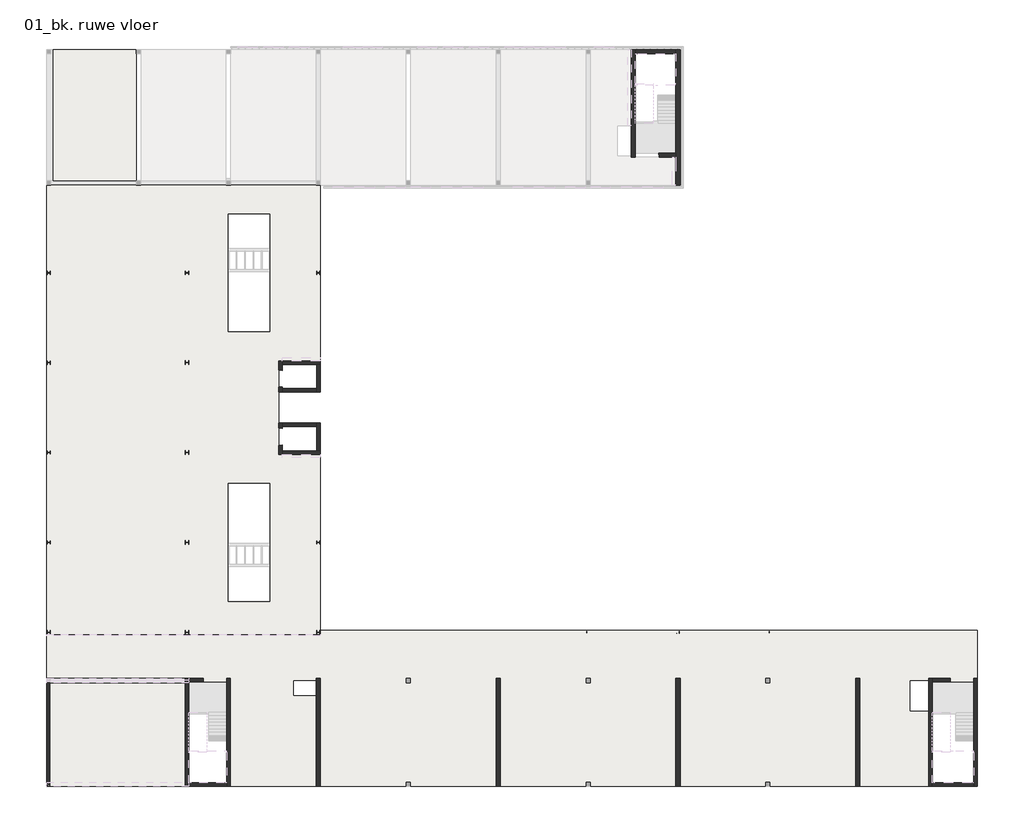
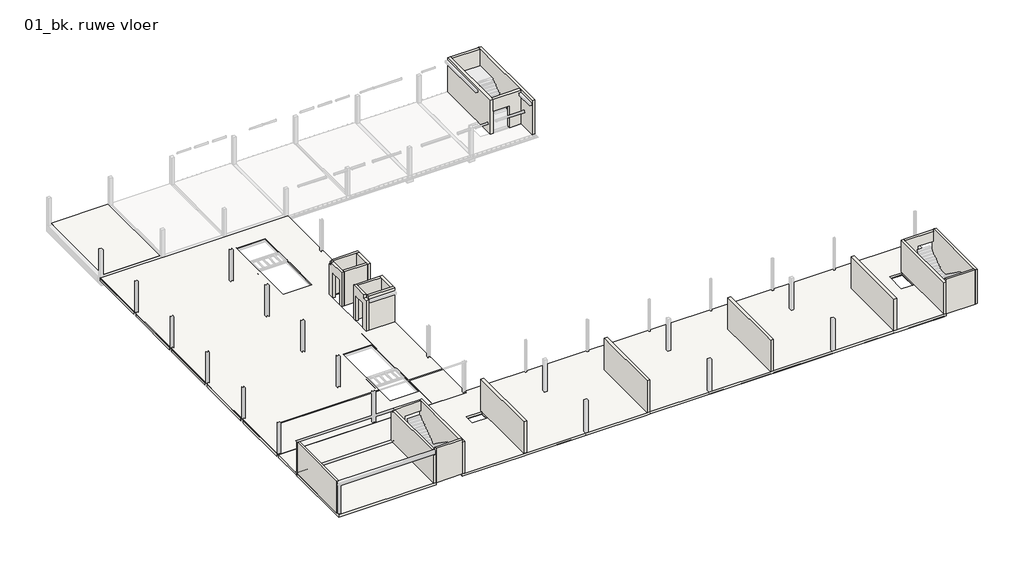
# One storey, part 1 of 4: 25 walls, 20 slabs.
"""IFC4 building model written with IfcOpenShell, lengths in millimetres."""

from ifc_helpers import new_model, si_unit, frame, origin, place, context, project, spatial, polyline, outline, extrude, faceted_brep, element, save

model = new_model("IFC4")

# Units and contexts
model_context = context("Model", 3, world=origin())
ifc_project = project(units=[si_unit("LENGTHUNIT", "METRE", prefix="MILLI")], contexts=[model_context])

# Site, building, storey
site = spatial("IfcSite", under=ifc_project)
building = spatial("IfcBuilding", under=site)
storey = spatial("IfcBuildingStorey", under=building, Name="01_bk. ruwe vloer", Elevation=3730.0)

# Slabs
placement = place(None, origin())
element("IfcSlab", 1, ObjectType="NLRS_23_FL_breedplaat 260_gen_rsf", at=placement, inside=storey, context=model_context, shape_type="Brep", body=[
    faceted_brep([(70375.0, -150.0, 3470.0), (70125.0, -150.0, 3470.0), (65200.0, -150.0, 3470.0), (64800.0, -150.0, 3470.0), (52200.0, -150.0, 3470.0), (51800.0, -150.0, 3470.0), (39200.0, -150.0, 3470.0), (38800.0, -150.0, 3470.0), (26200.0, -150.0, 3470.0), (25800.0, -150.0, 3470.0), (19625.0, -150.0, 3470.0), (19375.0, -150.0, 3470.0), (19375.0, 7400.0, 3470.0), (16625.0, 7400.0, 3470.0), (16625.0, 7493.0, 3470.0), (16625.0, 7507.0, 3470.0), (6350.0, 7507.0, 3470.0), (6350.0, 10845.0, 3470.0), (26125.0, 10845.0, 3470.0), (26125.0, 11125.0, 3470.0), (73650.0, 11125.0, 3470.0), (73650.0, 7400.0, 3470.0), (73400.0, 7400.0, 3470.0), (70375.0, 7400.0, 3470.0), (19600.0, 7622.0, 3470.0), (19600.0, -140.0, 3470.0), (25825.0, -140.0, 3470.0), (25825.0, 125.0, 3470.0), (26175.0, 125.0, 3470.0), (26175.0, -140.0, 3470.0), (32375.0, -140.0, 3470.0), (32375.0, 7625.0, 3470.0), (32625.0, 7625.0, 3470.0), (32625.0, -140.0, 3470.0), (38825.0, -140.0, 3470.0), (38825.0, 125.0, 3470.0), (39175.0, 125.0, 3470.0), (39175.0, -140.0, 3470.0), (45375.0, -140.0, 3470.0), (45375.0, 7625.0, 3470.0), (45625.0, 7625.0, 3470.0), (45625.0, -140.0, 3470.0), (51825.0, -140.0, 3470.0), (51825.0, 125.0, 3470.0), (52175.0, 125.0, 3470.0), (52175.0, -140.0, 3470.0), (58375.0, -140.0, 3470.0), (58375.0, 7625.0, 3470.0), (58625.0, 7625.0, 3470.0), (58625.0, -140.0, 3470.0), (64825.0, -140.0, 3470.0), (64825.0, 125.0, 3470.0), (65175.0, 125.0, 3470.0), (65175.0, -140.0, 3470.0), (70150.0, -140.0, 3470.0), (70150.0, 7625.0, 3470.0), (73640.0, 7625.0, 3470.0), (73640.0, 11115.0, 3470.0), (26135.0, 11115.0, 3470.0), (26135.0, 10750.0, 3470.0), (6360.0, 10750.0, 3470.0), (6360.0, 7622.0, 3470.0), (51825.0, 7625.0, 3470.0), (52175.0, 7625.0, 3470.0), (52175.0, 7375.0, 3470.0), (51825.0, 7375.0, 3470.0), (64825.0, 7625.0, 3470.0), (65175.0, 7625.0, 3470.0), (65175.0, 7375.0, 3470.0), (64825.0, 7375.0, 3470.0), (38825.0, 7625.0, 3470.0), (39175.0, 7625.0, 3470.0), (39175.0, 7375.0, 3470.0), (38825.0, 7375.0, 3470.0), (25850.0, 7375.0, 3470.0), (25850.0, 7500.0, 3470.0), (25825.0, 7500.0, 3470.0), (25825.0, 7625.0, 3470.0), (26175.0, 7625.0, 3470.0), (26175.0, 7375.0, 3470.0), (19375.0, -150.0, 3730.0), (19625.0, -150.0, 3730.0), (25850.0, -150.0, 3730.0), (26150.0, -150.0, 3730.0), (32350.0, -150.0, 3730.0), (32650.0, -150.0, 3730.0), (38850.0, -150.0, 3730.0), (39150.0, -150.0, 3730.0), (45350.0, -150.0, 3730.0), (45650.0, -150.0, 3730.0), (51850.0, -150.0, 3730.0), (52150.0, -150.0, 3730.0), (58350.0, -150.0, 3730.0), (58650.0, -150.0, 3730.0), (64850.0, -150.0, 3730.0), (65150.0, -150.0, 3730.0), (70125.0, -150.0, 3730.0), (70375.0, -150.0, 3730.0), (70375.0, 7400.0, 3730.0), (71700.0, 7400.0, 3730.0), (73650.0, 7400.0, 3730.0), (73650.0, 11125.0, 3730.0), (26125.0, 11125.0, 3730.0), (26125.0, 10845.0, 3730.0), (6350.0, 10845.0, 3730.0), (6350.0, 7507.0, 3730.0), (16625.0, 7507.0, 3730.0), (16625.0, 7493.0, 3730.0), (16625.0, 7400.0, 3730.0), (19375.0, 7400.0, 3730.0), (19375.0, 100.0, 3730.0), (24227.5, 6452.0, 3730.0), (24227.5, 7500.0, 3730.0), (25850.0, 7500.0, 3730.0), (25850.0, 6452.0, 3730.0), (68805.0, 5320.0, 3730.0), (68805.0, 7500.0, 3730.0), (70125.0, 7500.0, 3730.0), (70125.0, 5320.0, 3730.0), (6350.0, 10845.0, 3680.0), (26125.0, 10845.0, 3680.0), (19600.0, -140.0, 3530.0), (19600.0, 7622.0, 3530.0), (6360.0, 7622.0, 3530.0), (6360.0, 10750.0, 3530.0), (26135.0, 10750.0, 3530.0), (26135.0, 11115.0, 3530.0), (73640.0, 11115.0, 3530.0), (73640.0, 7625.0, 3530.0), (70150.0, 7625.0, 3530.0), (70150.0, -140.0, 3530.0), (65175.0, -140.0, 3530.0), (65175.0, 125.0, 3530.0), (64825.0, 125.0, 3530.0), (64825.0, -140.0, 3530.0), (58625.0, -140.0, 3530.0), (58625.0, 7625.0, 3530.0), (58375.0, 7625.0, 3530.0), (58375.0, -140.0, 3530.0), (52175.0, -140.0, 3530.0), (52175.0, 125.0, 3530.0), (51825.0, 125.0, 3530.0), (51825.0, -140.0, 3530.0), (45625.0, -140.0, 3530.0), (45625.0, 7625.0, 3530.0), (45375.0, 7625.0, 3530.0), (45375.0, -140.0, 3530.0), (39175.0, -140.0, 3530.0), (39175.0, 125.0, 3530.0), (38825.0, 125.0, 3530.0), (38825.0, -140.0, 3530.0), (32625.0, -140.0, 3530.0), (32625.0, 7625.0, 3530.0), (32375.0, 7625.0, 3530.0), (32375.0, -140.0, 3530.0), (26175.0, -140.0, 3530.0), (26175.0, 125.0, 3530.0), (25825.0, 125.0, 3530.0), (25825.0, -140.0, 3530.0), (26175.0, 7625.0, 3530.0), (25825.0, 7625.0, 3530.0), (25825.0, 7500.0, 3530.0), (24227.5, 7500.0, 3530.0), (24227.5, 6452.0, 3530.0), (25850.0, 6452.0, 3530.0), (25850.0, 7375.0, 3530.0), (26175.0, 7375.0, 3530.0), (52175.0, 7625.0, 3530.0), (51825.0, 7625.0, 3530.0), (51825.0, 7375.0, 3530.0), (52175.0, 7375.0, 3530.0), (65175.0, 7625.0, 3530.0), (64825.0, 7625.0, 3530.0), (64825.0, 7375.0, 3530.0), (65175.0, 7375.0, 3530.0), (39175.0, 7625.0, 3530.0), (38825.0, 7625.0, 3530.0), (38825.0, 7375.0, 3530.0), (39175.0, 7375.0, 3530.0), (68805.0, 7500.0, 3530.0), (68805.0, 5320.0, 3530.0), (70125.0, 5320.0, 3530.0), (70125.0, 7500.0, 3530.0)], [[[0, 1, 2, 3, 4, 5, 6, 7, 8, 9, 10, 11, 12, 13, 14, 15, 16, 17, 18, 19, 20, 21, 22, 23], [24, 25, 26, 27, 28, 29, 30, 31, 32, 33, 34, 35, 36, 37, 38, 39, 40, 41, 42, 43, 44, 45, 46, 47, 48, 49, 50, 51, 52, 53, 54, 55, 56, 57, 58, 59, 60, 61]], [[62, 63, 64, 65]], [[66, 67, 68, 69]], [[70, 71, 72, 73]], [[74, 75, 76, 77, 78, 79]], [[80, 81, 82, 83, 84, 85, 86, 87, 88, 89, 90, 91, 92, 93, 94, 95, 96, 97, 98, 99, 100, 101, 102, 103, 104, 105, 106, 107, 108, 109, 110], [111, 112, 113, 114], [115, 116, 117, 118]], [[11, 10, 9, 8, 7, 6, 5, 4, 3, 2, 1, 0, 97, 96, 95, 94, 93, 92, 91, 90, 89, 88, 87, 86, 85, 84, 83, 82, 81, 80]], [[12, 11, 80, 110, 109]], [[13, 12, 109, 108]], [[13, 108, 107, 106, 15, 14]], [[17, 16, 105, 104, 119]], [[18, 17, 119, 104, 103, 120]], [[19, 18, 120, 103, 102]], [[20, 19, 102, 101]], [[21, 20, 101, 100]], [[23, 22, 21, 100, 99, 98]], [[0, 23, 98, 97]], [[16, 15, 106, 105]], [[121, 122, 123, 124, 125, 126, 127, 128, 129, 130, 131, 132, 133, 134, 135, 136, 137, 138, 139, 140, 141, 142, 143, 144, 145, 146, 147, 148, 149, 150, 151, 152, 153, 154, 155, 156, 157, 158], [159, 160, 161, 162, 163, 164, 165, 166], [167, 168, 169, 170], [171, 172, 173, 174], [175, 176, 177, 178], [179, 180, 181, 182]], [[122, 121, 25, 24]], [[123, 122, 24, 61]], [[124, 123, 61, 60]], [[125, 124, 60, 59]], [[126, 125, 59, 58]], [[127, 126, 58, 57]], [[128, 127, 57, 56]], [[129, 128, 56, 55]], [[130, 129, 55, 54]], [[131, 130, 54, 53]], [[132, 131, 53, 52]], [[133, 132, 52, 51]], [[134, 133, 51, 50]], [[135, 134, 50, 49]], [[136, 135, 49, 48]], [[137, 136, 48, 47]], [[138, 137, 47, 46]], [[139, 138, 46, 45]], [[140, 139, 45, 44]], [[141, 140, 44, 43]], [[142, 141, 43, 42]], [[143, 142, 42, 41]], [[144, 143, 41, 40]], [[145, 144, 40, 39]], [[146, 145, 39, 38]], [[147, 146, 38, 37]], [[148, 147, 37, 36]], [[149, 148, 36, 35]], [[150, 149, 35, 34]], [[151, 150, 34, 33]], [[152, 151, 33, 32]], [[153, 152, 32, 31]], [[154, 153, 31, 30]], [[155, 154, 30, 29]], [[156, 155, 29, 28]], [[157, 156, 28, 27]], [[158, 157, 27, 26]], [[121, 158, 26, 25]], [[160, 159, 78, 77]], [[161, 160, 77, 76]], [[166, 165, 74, 79]], [[159, 166, 79, 78]], [[168, 167, 63, 62]], [[169, 168, 62, 65]], [[170, 169, 65, 64]], [[167, 170, 64, 63]], [[172, 171, 67, 66]], [[173, 172, 66, 69]], [[174, 173, 69, 68]], [[171, 174, 68, 67]], [[176, 175, 71, 70]], [[177, 176, 70, 73]], [[178, 177, 73, 72]], [[175, 178, 72, 71]], [[112, 111, 163, 162]], [[111, 114, 164, 163]], [[113, 75, 74, 165, 164, 114]], [[75, 113, 112, 162, 161, 76]], [[116, 115, 180, 179]], [[115, 118, 181, 180]], [[118, 117, 182, 181]], [[117, 116, 179, 182]]]),
])
element("IfcSlab", 2, ObjectType="NLRS_23_FL_breedplaat 260_gen_rsf", at=placement, inside=storey, context=model_context, shape_type="Brep", body=[
    faceted_brep([(6830.0, 43680.0, 3470.0), (6830.0, 43800.0, 3470.0), (6830.0, 53150.0, 3470.0), (6950.0, 53150.0, 3470.0), (12700.0, 53150.0, 3470.0), (12820.0, 53150.0, 3470.0), (12820.0, 43680.0, 3470.0), (12700.0, 43680.0, 3470.0), (12725.0, 43775.0, 3470.0), (12725.0, 53140.0, 3470.0), (6925.0, 53140.0, 3470.0), (6925.0, 43775.0, 3470.0), (6830.0, 53150.0, 3730.0), (6830.0, 43680.0, 3730.0), (12820.0, 43680.0, 3730.0), (12820.0, 53150.0, 3730.0), (6925.0, 53140.0, 3530.0), (12725.0, 53140.0, 3530.0), (12725.0, 43775.0, 3530.0), (6925.0, 43775.0, 3530.0)], [[[0, 1, 2, 3, 4, 5, 6, 7], [8, 9, 10, 11]], [[12, 13, 14, 15]], [[2, 1, 0, 13, 12]], [[5, 4, 3, 2, 12, 15]], [[6, 5, 15, 14]], [[0, 7, 6, 14, 13]], [[16, 17, 18, 19]], [[18, 17, 9, 8]], [[19, 18, 8, 11]], [[16, 19, 11, 10]], [[17, 16, 10, 9]]]),
])
element("IfcSlab", 3, ObjectType="NLRS_23_FL_druklaag 70_gen_rsf", at=placement, inside=storey, context=model_context, shape_type="Brep", body=[
    faceted_brep([(26125.0, 23875.0, 3660.0), (26125.0, 23795.0, 3660.0), (26125.0, 17675.0, 3660.0), (26125.0, 17655.0, 3660.0), (26125.0, 17345.0, 3660.0), (26125.0, 17325.0, 3660.0), (26125.0, 11175.0, 3660.0), (26125.0, 11155.0, 3660.0), (6350.0, 11155.0, 3660.0), (6350.0, 11175.0, 3660.0), (6350.0, 17325.0, 3660.0), (6350.0, 17345.0, 3660.0), (19240.0, 17345.0, 3660.0), (19240.0, 17655.0, 3660.0), (6350.0, 17655.0, 3660.0), (6350.0, 17675.0, 3660.0), (6350.0, 23825.0, 3660.0), (6350.0, 23845.0, 3660.0), (19240.0, 23845.0, 3660.0), (19500.0, 23845.0, 3660.0), (22500.0, 23845.0, 3660.0), (22760.0, 23845.0, 3660.0), (23362.3, 23845.0, 3660.0), (23362.3, 23875.0, 3660.0), (22500.0, 21750.0, 3660.0), (19500.0, 21750.0, 3660.0), (19500.0, 13250.0, 3660.0), (22500.0, 13250.0, 3660.0), (19500.0000006, 22062.0, 3660.0), (19500.0000006, 21760.0, 3660.0), (22499.9999994, 21760.0, 3660.0), (22499.9999994, 22062.0, 3660.0), (19500.0000006, 13240.0, 3660.0), (19500.0000006, 12938.0, 3660.0), (22499.9999994, 12938.0, 3660.0), (22499.9999994, 13240.0, 3660.0), (23125.0, 24155.0, 3660.0), (6350.0, 24155.0, 3660.0), (6350.0, 24175.0, 3660.0), (6350.0, 30302.0, 3660.0), (6350.0, 30322.0, 3660.0), (23125.0, 30322.0, 3660.0), (23125.0, 30302.0, 3660.0), (23125.0, 24175.0, 3660.0), (6350.0, 43350.0, 3660.0), (26125.0, 43350.0, 3660.0), (26125.0, 43330.0, 3660.0), (26125.0, 37175.0, 3660.0), (26125.0, 37155.0, 3660.0), (22760.0, 37155.0, 3660.0), (22760.0, 36845.0, 3660.0), (26125.0, 36845.0, 3660.0), (26125.0, 36825.0, 3660.0), (26125.0, 30705.0, 3660.0), (26125.0, 30625.0, 3660.0), (23362.3, 30625.0, 3660.0), (23362.3, 30632.0, 3660.0), (6350.0, 30632.0, 3660.0), (6350.0, 30652.0, 3660.0), (6350.0, 36825.0, 3660.0), (6350.0, 36845.0, 3660.0), (19240.0, 36845.0, 3660.0), (19240.0, 37155.0, 3660.0), (6350.0, 37155.0, 3660.0), (6350.0, 37175.0, 3660.0), (6350.0, 43330.0, 3660.0), (22500.0, 32750.0, 3660.0), (22500.0, 41250.0, 3660.0), (19500.0, 41250.0, 3660.0), (19500.0, 32750.0, 3660.0), (19500.0000006, 41562.0, 3660.0), (19500.0000006, 41260.0, 3660.0), (22499.9999994, 41260.0, 3660.0), (22499.9999994, 41562.0, 3660.0), (19500.0000006, 32740.0, 3660.0), (19500.0000006, 32438.0, 3660.0), (22499.9999994, 32438.0, 3660.0), (22499.9999994, 32740.0, 3660.0), (26125.0, 30625.0, 3730.0), (26125.0, 43350.0, 3730.0), (13180.0, 43350.0, 3730.0), (12820.0, 43350.0, 3730.0), (6350.0, 43350.0, 3730.0), (6350.0, 10845.0, 3730.0), (26125.0, 10845.0, 3730.0), (26125.0, 11125.0, 3730.0), (26125.0, 23875.0, 3730.0), (23125.0, 23875.0, 3730.0), (23125.0, 30625.0, 3730.0), (22500.0, 41250.0, 3730.0), (22500.0, 32750.0, 3730.0), (19500.0, 32750.0, 3730.0), (19500.0, 41250.0, 3730.0), (19500.0, 21750.0, 3730.0), (22500.0, 21750.0, 3730.0), (22500.0, 13250.0, 3730.0), (19500.0, 13250.0, 3730.0), (26125.0, 36845.0, 3680.0), (26125.0, 37155.0, 3680.0), (6350.0, 10845.0, 3680.0), (26125.0, 10845.0, 3680.0), (6350.0, 37155.0, 3680.0), (6350.0, 36845.0, 3680.0), (6350.0, 30632.0, 3680.0), (6350.0, 30322.0, 3680.0), (6350.0, 24155.0, 3680.0), (6350.0, 23845.0, 3680.0), (6350.0, 17655.0, 3680.0), (6350.0, 17345.0, 3680.0), (6350.0, 11155.0, 3680.0), (23125.0, 30625.0, 3680.0), (23362.3, 30625.0, 3680.0), (23125.0, 23875.0, 3680.0), (23125.0, 24155.0, 3680.0), (23125.0, 30322.0, 3680.0), (23362.3, 23875.0, 3680.0), (26125.0, 11125.0, 3680.0), (26125.0, 11155.0, 3680.0), (19240.0, 17345.0, 3680.0), (19240.0, 17655.0, 3680.0), (23362.3, 23845.0, 3680.0), (23362.3, 30632.0, 3680.0), (19240.0, 36845.0, 3680.0), (19240.0, 37155.0, 3680.0), (22760.0, 37155.0, 3680.0), (22760.0, 36845.0, 3680.0), (19500.0000006, 41562.0, 3680.0), (19500.0000006, 41260.0, 3680.0), (22499.9999994, 41260.0, 3680.0), (22499.9999994, 41562.0, 3680.0), (19500.0000006, 32740.0, 3680.0), (19500.0000006, 32438.0, 3680.0), (22499.9999994, 32438.0, 3680.0), (22499.9999994, 32740.0, 3680.0), (19500.0000006, 22062.0, 3680.0), (19500.0000006, 21760.0, 3680.0), (22499.9999994, 21760.0, 3680.0), (22499.9999994, 22062.0, 3680.0), (19500.0000006, 13240.0, 3680.0), (19500.0000006, 12938.0, 3680.0), (22499.9999994, 12938.0, 3680.0), (22499.9999994, 13240.0, 3680.0)], [[[0, 1, 2, 3, 4, 5, 6, 7, 8, 9, 10, 11, 12, 13, 14, 15, 16, 17, 18, 19, 20, 21, 22, 23], [24, 25, 26, 27], [28, 29, 30, 31], [32, 33, 34, 35]], [[36, 37, 38, 39, 40, 41, 42, 43]], [[44, 45, 46, 47, 48, 49, 50, 51, 52, 53, 54, 55, 56, 57, 58, 59, 60, 61, 62, 63, 64, 65], [66, 67, 68, 69], [70, 71, 72, 73], [74, 75, 76, 77]], [[78, 79, 80, 81, 82, 83, 84, 85, 86, 87, 88], [89, 90, 91, 92], [93, 94, 95, 96]], [[79, 78, 54, 53, 52, 51, 97, 98, 48, 47, 46, 45]], [[84, 83, 99, 100]], [[83, 82, 44, 65, 64, 63, 101, 102, 60, 59, 58, 57, 103, 104, 40, 39, 38, 37, 105, 106, 17, 16, 15, 14, 107, 108, 11, 10, 9, 8, 109, 99]], [[45, 44, 82, 81, 80, 79]], [[78, 88, 110, 111, 55, 54]], [[88, 87, 112, 113, 36, 43, 42, 41, 114, 110]], [[87, 86, 0, 23, 115, 112]], [[0, 86, 85, 84, 100, 116, 117, 7, 6, 5, 4, 3, 2, 1]], [[67, 66, 90, 89]], [[68, 67, 89, 92]], [[69, 68, 92, 91]], [[66, 69, 91, 90]], [[25, 24, 94, 93]], [[26, 25, 93, 96]], [[27, 26, 96, 95]], [[24, 27, 95, 94]], [[109, 117, 116, 100, 99]], [[117, 109, 8, 7]], [[118, 119, 13, 12]], [[119, 118, 108, 107]], [[119, 107, 14, 13]], [[108, 118, 12, 11]], [[120, 115, 23, 22]], [[120, 106, 105, 113, 112, 115]], [[113, 105, 37, 36]], [[106, 120, 22, 21, 20, 19, 18, 17]], [[111, 121, 56, 55]], [[103, 121, 111, 110, 114, 104]], [[121, 103, 57, 56]], [[104, 114, 41, 40]], [[122, 123, 62, 61]], [[123, 122, 102, 101]], [[123, 101, 63, 62]], [[102, 122, 61, 60]], [[124, 125, 50, 49]], [[125, 124, 98, 97]], [[98, 124, 49, 48]], [[125, 97, 51, 50]], [[126, 127, 71, 70]], [[128, 129, 73, 72]], [[127, 126, 129, 128]], [[127, 128, 72, 71]], [[129, 126, 70, 73]], [[130, 131, 75, 74]], [[132, 133, 77, 76]], [[131, 130, 133, 132]], [[133, 130, 74, 77]], [[131, 132, 76, 75]], [[134, 135, 29, 28]], [[136, 137, 31, 30]], [[135, 134, 137, 136]], [[135, 136, 30, 29]], [[137, 134, 28, 31]], [[138, 139, 33, 32]], [[140, 141, 35, 34]], [[139, 138, 141, 140]], [[141, 138, 32, 35]], [[139, 140, 34, 33]]]),
])
element("IfcSlab", 4, ObjectType="NLRS_23_FL_kanaalplaat 260_gen_rsf", at=placement, inside=storey, context=model_context, shape_type="SweptSolid", body=[
    extrude(outline(polyline([(19240.0, 11175.0), (6350.0, 11175.0), (6350.0, 17325.0), (19240.0, 17325.0), (19240.0, 11175.0)])), frame((0.0, 0.0, 3400.0), z_axis=(0.0, 0.0, 1.0), x_axis=(1.0, 0.0, 0.0)), (0.0, 0.0, 1.0), 260.0),
])
element("IfcSlab", 5, ObjectType="NLRS_23_FL_kanaalplaat 260_gen_rsf", at=placement, inside=storey, context=model_context, shape_type="SweptSolid", body=[
    extrude(outline(polyline([(6350.0, 17675.0), (6350.0, 23825.0), (19240.0, 23825.0), (19240.0, 17675.0), (6350.0, 17675.0)])), frame((0.0, 0.0, 3400.0), z_axis=(0.0, 0.0, 1.0), x_axis=(1.0, 0.0, 0.0)), (0.0, 0.0, 1.0), 260.0),
])
element("IfcSlab", 6, ObjectType="NLRS_23_FL_kanaalplaat 260_gen_rsf", at=placement, inside=storey, context=model_context, shape_type="SweptSolid", body=[
    extrude(outline(polyline([(23125.0, 30302.0), (23125.0, 24175.0), (6350.0, 24175.0), (6350.0, 30302.0), (23125.0, 30302.0)])), frame((0.0, 0.0, 3400.0), z_axis=(0.0, 0.0, 1.0), x_axis=(1.0, 0.0, 0.0)), (0.0, 0.0, 1.0), 260.0),
])
element("IfcSlab", 7, ObjectType="NLRS_23_FL_kanaalplaat 260_gen_rsf", at=placement, inside=storey, context=model_context, shape_type="SweptSolid", body=[
    extrude(outline(polyline([(22500.0, 23825.0), (22500.0, 22082.0), (19500.0, 22082.0), (19500.0, 23825.0), (22500.0, 23825.0)])), frame((0.0, 0.0, 3400.0), z_axis=(0.0, 0.0, 1.0), x_axis=(1.0, 0.0, 0.0)), (0.0, 0.0, 1.0), 260.0),
])
element("IfcSlab", 8, ObjectType="NLRS_23_FL_kanaalplaat 260_gen_rsf", at=placement, inside=storey, context=model_context, shape_type="SweptSolid", body=[
    extrude(outline(polyline([(22500.0, 11182.5), (19500.0, 11182.5), (19500.0, 12918.0), (22500.0, 12918.0), (22500.0, 11182.5)])), frame((0.0, 0.0, 3400.0), z_axis=(0.0, 0.0, 1.0), x_axis=(1.0, 0.0, 0.0)), (0.0, 0.0, 1.0), 260.0),
])
element("IfcSlab", 9, ObjectType="NLRS_23_FL_kanaalplaat 260_gen_rsf", at=placement, inside=storey, context=model_context, shape_type="Brep", body=[
    faceted_brep([(26125.0, 23795.0, 3400.0), (26125.0, 23625.0, 3400.0), (26125.0, 17675.0, 3400.0), (22760.0, 17675.0, 3400.0), (22760.0, 23825.0, 3400.0), (23395.0, 23825.0, 3400.0), (23395.0, 23795.0, 3400.0), (26125.0, 23795.0, 3660.0), (23395.0, 23795.0, 3660.0), (23395.0, 23825.0, 3660.0), (22760.0, 23825.0, 3660.0), (22760.0, 17675.0, 3660.0), (26125.0, 17675.0, 3660.0)], [[[0, 1, 2, 3, 4, 5, 6]], [[7, 8, 9, 10, 11, 12]], [[2, 1, 0, 7, 12]], [[3, 2, 12, 11]], [[4, 3, 11, 10]], [[5, 4, 10, 9]], [[6, 5, 9, 8]], [[0, 6, 8, 7]]]),
])
element("IfcSlab", 10, ObjectType="NLRS_23_FL_kanaalplaat 260_gen_rsf", at=placement, inside=storey, context=model_context, shape_type="SweptSolid", body=[
    extrude(outline(polyline([(22760.0, 11175.0), (22760.0, 17325.0), (26125.0, 17325.0), (26125.0, 11175.0), (22760.0, 11175.0)])), frame((0.0, 0.0, 3400.0), z_axis=(0.0, 0.0, 1.0), x_axis=(1.0, 0.0, 0.0)), (0.0, 0.0, 1.0), 260.0),
])
element("IfcSlab", 11, ObjectType="NLRS_23_FL_kanaalplaat 260_gen_rsf", at=placement, inside=storey, context=model_context, shape_type="Brep", body=[
    faceted_brep([(19240.0, 43330.0, 3400.0), (19240.0, 37175.0, 3400.0), (6350.0, 37175.0, 3400.0), (6350.0, 43200.0, 3400.0), (6350.0, 43330.0, 3400.0), (19240.0, 43330.0, 3660.0), (6350.0, 43330.0, 3660.0), (6350.0, 37175.0, 3660.0), (19240.0, 37175.0, 3660.0)], [[[0, 1, 2, 3, 4]], [[5, 6, 7, 8]], [[0, 4, 6, 5]], [[4, 3, 2, 7, 6]], [[2, 1, 8, 7]], [[1, 0, 5, 8]]]),
])
element("IfcSlab", 12, ObjectType="NLRS_23_FL_kanaalplaat 260_gen_rsf", at=placement, inside=storey, context=model_context, shape_type="SweptSolid", body=[
    extrude(outline(polyline([(6350.0, 36825.0), (19240.0, 36825.0), (19240.0, 30652.0), (6350.0, 30652.0), (6350.0, 36825.0)])), frame((0.0, 0.0, 3400.0), z_axis=(0.0, 0.0, 1.0), x_axis=(1.0, 0.0, 0.0)), (0.0, 0.0, 1.0), 260.0),
])
element("IfcSlab", 13, ObjectType="NLRS_23_FL_kanaalplaat 260_gen_rsf", at=placement, inside=storey, context=model_context, shape_type="SweptSolid", body=[
    extrude(outline(polyline([(22500.0, 30652.0), (19500.0, 30652.0), (19500.0, 32418.0), (22500.0, 32418.0), (22500.0, 30652.0)])), frame((0.0, 0.0, 3400.0), z_axis=(0.0, 0.0, 1.0), x_axis=(1.0, 0.0, 0.0)), (0.0, 0.0, 1.0), 260.0),
])
element("IfcSlab", 14, ObjectType="NLRS_23_FL_kanaalplaat 260_gen_rsf", at=placement, inside=storey, context=model_context, shape_type="SweptSolid", body=[
    extrude(outline(polyline([(22500.0, 43330.0), (22500.0, 41582.0), (19500.0, 41582.0), (19500.0, 43330.0), (22500.0, 43330.0)])), frame((0.0, 0.0, 3400.0), z_axis=(0.0, 0.0, 1.0), x_axis=(1.0, 0.0, 0.0)), (0.0, 0.0, 1.0), 260.0),
])
element("IfcSlab", 15, ObjectType="NLRS_23_FL_kanaalplaat 260_gen_rsf", at=placement, inside=storey, context=model_context, shape_type="Brep", body=[
    faceted_brep([(26125.0, 30705.0, 3400.0), (23395.0, 30705.0, 3400.0), (23395.0, 30652.0, 3400.0), (22760.0, 30652.0, 3400.0), (22760.0, 36825.0, 3400.0), (26125.0, 36825.0, 3400.0), (26125.0, 30875.0, 3400.0), (26125.0, 30705.0, 3660.0), (26125.0, 36825.0, 3660.0), (22760.0, 36825.0, 3660.0), (22760.0, 30652.0, 3660.0), (23395.0, 30652.0, 3660.0), (23395.0, 30705.0, 3660.0)], [[[0, 1, 2, 3, 4, 5, 6]], [[7, 8, 9, 10, 11, 12]], [[0, 6, 5, 8, 7]], [[5, 4, 9, 8]], [[4, 3, 10, 9]], [[3, 2, 11, 10]], [[2, 1, 12, 11]], [[1, 0, 7, 12]]]),
])
element("IfcSlab", 16, ObjectType="NLRS_23_FL_kanaalplaat 260_gen_rsf", at=placement, inside=storey, context=model_context, shape_type="Brep", body=[
    faceted_brep([(22760.0, 43330.0, 3400.0), (26125.0, 43330.0, 3400.0), (26125.0, 43200.0, 3400.0), (26125.0, 37175.0, 3400.0), (22760.0, 37175.0, 3400.0), (22760.0, 43330.0, 3660.0), (22760.0, 37175.0, 3660.0), (26125.0, 37175.0, 3660.0), (26125.0, 43330.0, 3660.0)], [[[0, 1, 2, 3, 4]], [[5, 6, 7, 8]], [[0, 4, 6, 5]], [[4, 3, 7, 6]], [[3, 2, 1, 8, 7]], [[1, 0, 5, 8]]]),
])
element("IfcSlab", 17, ObjectType="NLRS_23_FL_breedplaat 260_gen_rsf", at=placement, inside=storey, context=model_context, shape_type="Brep", body=[
    faceted_brep([(6350.0, -150.0, 3470.0), (6350.0, 7493.0, 3470.0), (16625.0, 7493.0, 3470.0), (16625.0, -150.0, 3470.0), (6539.0, 125.0, 3470.0), (16400.0, 125.0, 3470.0), (16400.0, 7378.0, 3470.0), (6539.0, 7378.0, 3470.0), (6350.0, 7493.0, 3730.0), (6350.0, -150.0, 3730.0), (16375.0, -150.0, 3730.0), (16625.0, -150.0, 3730.0), (16625.0, 100.0, 3730.0), (16625.0, 7493.0, 3730.0), (16400.0, 7378.0, 3530.0), (16400.0, 125.0, 3530.0), (6539.0, 125.0, 3530.0), (6539.0, 7378.0, 3530.0)], [[[0, 1, 2, 3], [4, 5, 6, 7]], [[8, 9, 10, 11, 12, 13]], [[1, 0, 9, 8]], [[2, 1, 8, 13]], [[3, 2, 13, 12, 11]], [[0, 3, 11, 10, 9]], [[14, 15, 16, 17]], [[16, 15, 5, 4]], [[17, 16, 4, 7]], [[14, 17, 7, 6]], [[15, 14, 6, 5]]]),
])
element("IfcSlab", 18, ObjectType="NLRS_23_FL_breedplaat schil 60_gen_rsf", at=placement, inside=storey, context=model_context, shape_type="SweptSolid", body=[
    extrude(outline(polyline([(16400.0, 125.0), (6539.0, 125.0), (6539.0, 7378.0), (16400.0, 7378.0), (16400.0, 125.0)])), frame((0.0, 0.0, 3470.0), z_axis=(0.0, 0.0, 1.0), x_axis=(1.0, 0.0, 0.0)), (0.0, 0.0, 1.0), 60.0),
])
element("IfcSlab", 19, ObjectType="NLRS_23_FL_breedplaat schil 60_gen_rsf", at=placement, inside=storey, context=model_context, shape_type="SweptSolid", body=[
    extrude(outline(polyline([(19600.0, -140.0), (19600.0, 7622.0), (6360.0, 7622.0), (6360.0, 10750.0), (26135.0, 10750.0), (26135.0, 11115.0), (73640.0, 11115.0), (73640.0, 7625.0), (70150.0, 7625.0), (70150.0, -140.0), (65175.0, -140.0), (65175.0, 125.0), (64825.0, 125.0), (64825.0, -140.0), (58625.0, -140.0), (58625.0, 7625.0), (58375.0, 7625.0), (58375.0, -140.0), (52175.0, -140.0), (52175.0, 125.0), (51825.0, 125.0), (51825.0, -140.0), (45625.0, -140.0), (45625.0, 7625.0), (45375.0, 7625.0), (45375.0, -140.0), (39175.0, -140.0), (39175.0, 125.0), (38825.0, 125.0), (38825.0, -140.0), (32625.0, -140.0), (32625.0, 7625.0), (32375.0, 7625.0), (32375.0, -140.0), (26175.0, -140.0), (26175.0, 125.0), (25825.0, 125.0), (25825.0, -140.0), (19600.0, -140.0)]), holes=[polyline([(26175.0, 7625.0), (25825.0, 7625.0), (25825.0, 7500.0), (24227.5, 7500.0), (24227.5, 6452.0), (25850.0, 6452.0), (25850.0, 7375.0), (26175.0, 7375.0), (26175.0, 7625.0)]), polyline([(52175.0, 7625.0), (51825.0, 7625.0), (51825.0, 7375.0), (52175.0, 7375.0), (52175.0, 7625.0)]), polyline([(65175.0, 7625.0), (64825.0, 7625.0), (64825.0, 7375.0), (65175.0, 7375.0), (65175.0, 7625.0)]), polyline([(39175.0, 7625.0), (38825.0, 7625.0), (38825.0, 7375.0), (39175.0, 7375.0), (39175.0, 7625.0)]), polyline([(68805.0, 7500.0), (68805.0, 5320.0), (70125.0, 5320.0), (70125.0, 7500.0), (68805.0, 7500.0)])]), frame((0.0, 0.0, 3470.0), z_axis=(0.0, 0.0, 1.0), x_axis=(1.0, 0.0, 0.0)), (0.0, 0.0, 1.0), 60.0),
])
element("IfcSlab", 20, ObjectType="NLRS_23_FL_breedplaat schil 60_gen_rsf", at=placement, inside=storey, context=model_context, shape_type="SweptSolid", body=[
    extrude(outline(polyline([(12725.0, 53140.0), (12725.0, 43775.0), (6925.0, 43775.0), (6925.0, 53140.0), (12725.0, 53140.0)])), frame((0.0, 0.0, 3470.0), z_axis=(0.0, 0.0, 1.0), x_axis=(1.0, 0.0, 0.0)), (0.0, 0.0, 1.0), 60.0),
])

# Walls
element("IfcWall", 21, ObjectType="NLRS_22_WA_beton ihw 250_gen_rsf", at=placement, inside=storey, context=model_context, shape_type="Brep", body=[
    faceted_brep([(19625.0, -150.0, 3730.0), (19625.0, 7650.0, 3730.0), (19625.0, 7650.0, 7270.0), (19625.0, -150.0, 7270.0), (19375.0, -150.0, 3730.0), (19375.0, -150.0, 7270.0), (19375.0, 7400.0, 7270.0), (19375.0, 7650.0, 7270.0), (19375.0, 7650.0, 6170.0), (19375.0, 7650.0, 3730.0), (19375.0, 7400.0, 3730.0), (19375.0, 100.0, 3730.0)], [[[0, 1, 2, 3]], [[4, 5, 6, 7, 8, 9, 10, 11]], [[1, 0, 4, 11, 10, 9]], [[2, 1, 9, 8, 7]], [[3, 2, 7, 6, 5]], [[0, 3, 5, 4]]]),
])
element("IfcWall", 22, ObjectType="NLRS_22_WA_beton ihw 250_gen_rsf", at=placement, inside=storey, context=model_context, shape_type="Brep", body=[
    faceted_brep([(16625.0, -150.0, 3730.0), (16625.0, 100.0, 3730.0), (16625.0, 7400.0, 3730.0), (16625.0, 7493.0, 3730.0), (16625.0, 7650.0, 3730.0), (16625.0, 7650.0, 7120.0), (16625.0, 7330.0, 7120.0), (16625.0, 7330.0, 7270.0), (16625.0, 170.0, 7270.0), (16625.0, 170.0, 6880.0), (16625.0, -150.0, 6880.0), (16375.0, -150.0, 3730.0), (16375.0, -150.0, 6880.0), (16375.0, 170.0, 6880.0), (16375.0, 170.0, 7270.0), (16375.0, 7330.0, 7270.0), (16375.0, 7330.0, 7120.0), (16375.0, 7650.0, 7120.0), (16375.0, 7650.0, 3730.0)], [[[0, 1, 2, 3, 4, 5, 6, 7, 8, 9, 10]], [[11, 12, 13, 14, 15, 16, 17, 18]], [[4, 3, 2, 1, 0, 11, 18]], [[5, 4, 18, 17]], [[8, 7, 15, 14]], [[0, 10, 12, 11]], [[6, 5, 17, 16]], [[7, 6, 16, 15]], [[9, 8, 14, 13]], [[10, 9, 13, 12]]]),
])
element("IfcWall", 23, ObjectType="NLRS_22_WA_beton ihw 300_gen_rsf", at=placement, inside=storey, context=model_context, shape_type="Brep", body=[
    faceted_brep([(26150.0, -150.0, 3730.0), (26150.0, 7650.0, 3730.0), (26150.0, 7650.0, 7270.0), (26150.0, -150.0, 7270.0), (25850.0, -150.0, 3730.0), (25850.0, -150.0, 7270.0), (25850.0, 7650.0, 7270.0), (25850.0, 7650.0, 3730.0), (25850.0, 7500.0, 3730.0), (25850.0, 6452.0, 3730.0)], [[[0, 1, 2, 3]], [[4, 5, 6, 7, 8, 9]], [[1, 0, 4, 9, 8, 7]], [[2, 1, 7, 6]], [[3, 2, 6, 5]], [[0, 3, 5, 4]]]),
])
element("IfcWall", 24, ObjectType="NLRS_22_WA_beton ihw 300_gen_rsf", at=placement, inside=storey, context=model_context, shape_type="SweptSolid", body=[
    extrude(outline(polyline([(39150.0, 7650.0), (39150.0, -150.0), (38850.0, -150.0), (38850.0, 7650.0), (39150.0, 7650.0)])), frame((0.0, 0.0, 3730.0), z_axis=(0.0, 0.0, 1.0), x_axis=(1.0, 0.0, 0.0)), (0.0, 0.0, 1.0), 3540.0),
])
element("IfcWall", 25, ObjectType="NLRS_22_WA_beton ihw 300_gen_rsf", at=placement, inside=storey, context=model_context, shape_type="SweptSolid", body=[
    extrude(outline(polyline([(52150.0, 7650.0), (52150.0, -150.0), (51850.0, -150.0), (51850.0, 7650.0), (52150.0, 7650.0)])), frame((0.0, 0.0, 3730.0), z_axis=(0.0, 0.0, 1.0), x_axis=(1.0, 0.0, 0.0)), (0.0, 0.0, 1.0), 3540.0),
])
element("IfcWall", 26, ObjectType="NLRS_22_WA_beton ihw 300_gen_rsf", at=placement, inside=storey, context=model_context, shape_type="SweptSolid", body=[
    extrude(outline(polyline([(65150.0, 7650.0), (65150.0, -150.0), (64850.0, -150.0), (64850.0, 7650.0), (65150.0, 7650.0)])), frame((0.0, 0.0, 3730.0), z_axis=(0.0, 0.0, 1.0), x_axis=(1.0, 0.0, 0.0)), (0.0, 0.0, 1.0), 3540.0),
])
element("IfcWall", 27, ObjectType="NLRS_21_WA_beton ihw 250_gen_rsf", at=placement, inside=storey, context=model_context, shape_type="Brep", body=[
    faceted_brep([(73650.0, -150.0, 3730.0), (73650.0, 7400.0, 3730.0), (73650.0, 7650.0, 3730.0), (73650.0, 7650.0, 7270.0), (73650.0, 7400.0, 7270.0), (73650.0, 7400.0, 7530.0), (73650.0, -150.0, 7530.0), (73400.0, -150.0, 3730.0), (73400.0, -150.0, 7530.0), (73400.0, 100.0, 7530.0), (73400.0, 7400.0, 7530.0), (73400.0, 7400.0, 7270.0), (73400.0, 7650.0, 7270.0), (73400.0, 7650.0, 6170.0), (73400.0, 7650.0, 3730.0), (73400.0, 7400.0, 3730.0), (73400.0, 100.0, 3730.0)], [[[0, 1, 2, 3, 4, 5, 6]], [[7, 8, 9, 10, 11, 12, 13, 14, 15, 16]], [[2, 1, 0, 7, 16, 15, 14]], [[3, 2, 14, 13, 12]], [[6, 5, 10, 9, 8]], [[0, 6, 8, 7]], [[4, 3, 12, 11]], [[5, 4, 11, 10]]]),
])
element("IfcWall", 28, ObjectType="NLRS_21_WA_kalkzandsteen CS12 214_gen_rsf", at=placement, inside=storey, context=model_context, shape_type="SweptSolid", body=[
    extrude(outline(polyline([(6564.0, 7330.0), (6564.0, 170.0), (6350.0, 170.0), (6350.0, 7330.0), (6564.0, 7330.0)])), frame((0.0, 0.0, 3730.0), z_axis=(0.0, 0.0, 1.0), x_axis=(1.0, 0.0, 0.0)), (0.0, 0.0, 1.0), 3540.0),
])
element("IfcWall", 29, ObjectType="NLRS_21_WA_beton ihw 250_gen_rsf", at=placement, inside=storey, context=model_context, shape_type="Brep", body=[
    faceted_brep([(16625.0, -150.0, 3730.0), (19375.0, -150.0, 3730.0), (19375.0, -150.0, 7270.0), (19375.0, -150.0, 7530.0), (16625.0, -150.0, 7530.0), (16625.0, -150.0, 7270.0), (16625.0, -150.0, 6880.0), (19375.0, 100.0, 3730.0), (16625.0, 100.0, 3730.0), (16625.0, 100.0, 7530.0), (19375.0, 100.0, 7530.0), (19375.0, 100.0, 7270.0)], [[[0, 1, 2, 3, 4, 5, 6]], [[7, 8, 9, 10, 11]], [[1, 0, 8, 7]], [[1, 7, 11, 10, 3, 2]], [[4, 3, 10, 9]], [[0, 6, 5, 4, 9, 8]]]),
])
element("IfcWall", 30, ObjectType="NLRS_22_WA_beton ihw 250_gen_rsf", at=placement, inside=storey, context=model_context, shape_type="Brep", body=[
    faceted_brep([(19375.0, 7400.0, 7270.0), (16625.0, 7400.0, 7270.0), (16625.0, 7400.0, 3730.0), (17675.0, 7400.0, 3730.0), (17675.0, 7400.0, 6170.0), (19375.0, 7400.0, 6170.0), (16625.0, 7650.0, 7270.0), (19375.0, 7650.0, 7270.0), (19375.0, 7650.0, 6170.0), (17675.0, 7650.0, 6170.0), (17675.0, 7650.0, 3730.0), (16625.0, 7650.0, 3730.0), (16625.0, 7650.0, 7120.0)], [[[0, 1, 2, 3, 4, 5]], [[6, 7, 8, 9, 10, 11, 12]], [[2, 11, 10, 3]], [[7, 0, 5, 8]], [[1, 0, 7, 6]], [[2, 1, 6, 12, 11]], [[9, 4, 3, 10]], [[4, 9, 8, 5]]]),
])
element("IfcWall", 31, ObjectType="NLRS_22_WA_beton ihw 250_gen_rsf", at=placement, inside=storey, context=model_context, shape_type="Brep", body=[
    faceted_brep([(70375.0, -150.0, 3730.0), (70375.0, 100.0, 3730.0), (70375.0, 7400.0, 3730.0), (70375.0, 7650.0, 3730.0), (70375.0, 7650.0, 7270.0), (70375.0, 7400.0, 7270.0), (70375.0, -150.0, 7270.0), (70125.0, -150.0, 3730.0), (70125.0, -150.0, 7270.0), (70125.0, 7650.0, 7270.0), (70125.0, 7650.0, 3730.0), (70125.0, 7500.0, 3730.0), (70125.0, 5320.0, 3730.0)], [[[0, 1, 2, 3, 4, 5, 6]], [[7, 8, 9, 10, 11, 12]], [[3, 2, 1, 0, 7, 12, 11, 10]], [[4, 3, 10, 9]], [[6, 5, 4, 9, 8]], [[0, 6, 8, 7]]]),
])
element("IfcWall", 32, ObjectType="NLRS_21_WA_beton ihw 250_gen_rsf", at=placement, inside=storey, context=model_context, shape_type="Brep", body=[
    faceted_brep([(70375.0, -150.0, 3730.0), (73400.0, -150.0, 3730.0), (73400.0, -150.0, 7530.0), (70375.0, -150.0, 7530.0), (70375.0, -150.0, 7270.0), (70375.0, 100.0, 3730.0), (70375.0, 100.0, 7530.0), (73400.0, 100.0, 7530.0), (73400.0, 100.0, 3730.0)], [[[0, 1, 2, 3, 4]], [[5, 6, 7, 8]], [[1, 0, 5, 8]], [[2, 1, 8, 7]], [[3, 2, 7, 6]], [[0, 4, 3, 6, 5]]]),
])
element("IfcWall", 33, ObjectType="NLRS_22_WA_beton ihw 250_gen_rsf", at=placement, inside=storey, context=model_context, shape_type="SweptSolid", body=[
    extrude(outline(polyline([(7270.0, 73400.0), (7270.0, 70375.0), (3730.0, 70375.0), (3730.0, 71700.0), (6170.0, 71700.0), (6170.0, 73400.0), (7270.0, 73400.0)])), frame((0.0, 7400.0, 0.0), z_axis=(0.0, 1.0, 0.0), x_axis=(0.0, 0.0, 1.0)), (0.0, 0.0, 1.0), 250.0),
])
element("IfcWall", 34, ObjectType="NLRS_22_WA_beton prefab 300_gen_rsf", at=placement, inside=storey, context=model_context, shape_type="Brep", body=[
    faceted_brep([(48905.0, 45350.0, 3750.0), (48905.0, 53150.0, 3750.0), (48905.0, 53150.0, 7530.0), (48905.0, 45350.0, 7530.0), (48605.0, 45350.0, 3750.0), (48605.0, 45350.0, 7530.0), (48605.0, 53150.0, 7530.0), (48605.0, 53150.0, 7270.0), (48605.0, 53150.0, 7020.0), (48605.0, 53150.0, 3750.0)], [[[0, 1, 2, 3]], [[4, 5, 6, 7, 8, 9]], [[1, 0, 4, 9]], [[2, 1, 9, 8, 7, 6]], [[3, 2, 6, 5]], [[0, 3, 5, 4]]]),
])
element("IfcWall", 35, ObjectType="NLRS_21_WA_beton prefab 300_gen_rsf", at=placement, inside=storey, context=model_context, shape_type="Brep", body=[
    faceted_brep([(52150.0, 43350.0, 3750.0), (52150.0, 53150.0, 3750.0), (52150.0, 53150.0, 7530.0), (52150.0, 43350.0, 7530.0), (51850.0, 43350.0, 3750.0), (51850.0, 43350.0, 7020.0), (51850.0, 43350.0, 7270.0), (51850.0, 43350.0, 7530.0), (51850.0, 53150.0, 7530.0), (51850.0, 53150.0, 3750.0)], [[[0, 1, 2, 3]], [[4, 5, 6, 7, 8, 9]], [[1, 0, 4, 9]], [[2, 1, 9, 8]], [[3, 2, 8, 7]], [[0, 3, 7, 6, 5, 4]]]),
])
element("IfcWall", 36, ObjectType="NLRS_21_WA_beton prefab 300_gen_rsf", at=placement, inside=storey, context=model_context, shape_type="SweptSolid", body=[
    extrude(outline(polyline([(48925.0, 53150.0), (51830.0, 53150.0), (51830.0, 52850.0), (48925.0, 52850.0), (48925.0, 53150.0)])), frame((0.0, 0.0, 3750.0), z_axis=(0.0, 0.0, 1.0), x_axis=(1.0, 0.0, 0.0)), (0.0, 0.0, 1.0), 3780.0),
])
element("IfcWall", 37, ObjectType="NLRS_22_WA_beton prefab 300_gen_rsf", at=placement, inside=storey, context=model_context, shape_type="Brep", body=[
    faceted_brep([(48925.0, 45650.0, 7530.0), (51830.0, 45650.0, 7530.0), (51830.0, 45650.0, 3750.0), (50625.0, 45650.0, 3750.0), (50625.0, 45650.0, 6170.0), (48925.0, 45650.0, 6170.0), (51830.0, 45350.0, 7530.0), (48925.0, 45350.0, 7530.0), (48925.0, 45350.0, 6200.0), (50655.0, 45350.0, 6200.0), (50655.0, 45350.0, 3750.0), (51830.0, 45350.0, 3750.0)], [[[0, 1, 2, 3, 4, 5]], [[6, 7, 8, 9, 10, 11]], [[2, 11, 10, 3]], [[7, 0, 5, 8]], [[1, 0, 7, 6]], [[2, 1, 6, 11]], [[9, 4, 3, 10]], [[4, 9, 8, 5]]]),
])
element("IfcWall", 38, ObjectType="NLRS_22_WA_beton prefab 250_gen_rsf", at=placement, inside=storey, context=model_context, shape_type="Brep", body=[
    faceted_brep([(26125.0, 30625.0, 3750.0), (23395.0, 30625.0, 3750.0), (23395.0, 30625.0, 6950.0), (23395.0, 30625.0, 7200.0), (23395.0, 30625.0, 7530.0), (26125.0, 30625.0, 7530.0), (26125.0, 30625.0, 7200.0), (26125.0, 30625.0, 6950.0), (26125.0, 30375.0, 3750.0), (26125.0, 30375.0, 7530.0), (23395.0, 30375.0, 7530.0), (23395.0, 30375.0, 3750.0)], [[[0, 1, 2, 3, 4, 5, 6, 7]], [[8, 9, 10, 11]], [[1, 0, 8, 11]], [[4, 3, 2, 1, 11, 10]], [[5, 4, 10, 9]], [[0, 7, 6, 5, 9, 8]]]),
])
element("IfcWall", 39, ObjectType="NLRS_22_WA_beton prefab 250_gen_rsf", at=placement, inside=storey, context=model_context, shape_type="Brep", body=[
    faceted_brep([(23125.0, 28375.0, 3750.0), (23125.0, 28375.0, 7530.0), (23125.0, 30231.5, 7530.0), (23125.0, 30231.5, 7155.0), (23125.0, 30625.0, 7155.0), (23125.0, 30625.0, 3750.0), (23125.0, 29973.0, 3750.0), (23125.0, 29973.0, 6505.0), (23125.0, 28723.0, 6505.0), (23125.0, 28723.0, 3750.0), (23375.0, 28375.0, 7530.0), (23375.0, 28375.0, 3750.0), (23375.0, 28748.0, 3750.0), (23375.0, 28748.0, 6480.0), (23375.0, 29948.0, 6480.0), (23375.0, 29948.0, 3750.0), (23375.0, 30625.0, 3750.0), (23375.0, 30625.0, 7155.0), (23375.0, 30231.5, 7155.0), (23375.0, 30231.5, 7530.0)], [[[0, 1, 2, 3, 4, 5, 6, 7, 8, 9]], [[10, 11, 12, 13, 14, 15, 16, 17, 18, 19]], [[11, 0, 9, 12]], [[5, 16, 15, 6]], [[1, 0, 11, 10]], [[2, 1, 10, 19]], [[5, 4, 17, 16]], [[3, 2, 19, 18]], [[4, 3, 18, 17]], [[14, 7, 6, 15]], [[8, 13, 12, 9]], [[7, 14, 13, 8]]]),
])
element("IfcWall", 40, ObjectType="NLRS_22_WA_beton prefab 250_gen_rsf", at=placement, inside=storey, context=model_context, shape_type="SweptSolid", body=[
    extrude(outline(polyline([(25855.0, 28375.0), (23395.0, 28375.0), (23395.0, 28625.0), (25855.0, 28625.0), (25855.0, 28375.0)])), frame((0.0, 0.0, 3750.0), z_axis=(0.0, 0.0, 1.0), x_axis=(1.0, 0.0, 0.0)), (0.0, 0.0, 1.0), 3780.0),
])
element("IfcWall", 41, ObjectType="NLRS_21_WA_beton prefab 250_gen_rsf", at=placement, inside=storey, context=model_context, shape_type="SweptSolid", body=[
    extrude(outline(polyline([(26125.0, 30355.0), (26125.0, 28375.0), (25875.0, 28375.0), (25875.0, 30355.0), (26125.0, 30355.0)])), frame((0.0, 0.0, 3750.0), z_axis=(0.0, 0.0, 1.0), x_axis=(1.0, 0.0, 0.0)), (0.0, 0.0, 1.0), 3780.0),
])
element("IfcWall", 42, ObjectType="NLRS_22_WA_beton prefab 250_gen_rsf", at=placement, inside=storey, context=model_context, shape_type="SweptSolid", body=[
    extrude(outline(polyline([(23395.0, 26125.0), (25855.0, 26125.0), (25855.0, 25875.0), (23395.0, 25875.0), (23395.0, 26125.0)])), frame((0.0, 0.0, 3750.0), z_axis=(0.0, 0.0, 1.0), x_axis=(1.0, 0.0, 0.0)), (0.0, 0.0, 1.0), 3780.0),
])
element("IfcWall", 43, ObjectType="NLRS_22_WA_beton prefab 250_gen_rsf", at=placement, inside=storey, context=model_context, shape_type="Brep", body=[
    faceted_brep([(23125.0, 23875.0, 3750.0), (23125.0, 23875.0, 7155.0), (23125.0, 24291.5, 7155.0), (23125.0, 24291.5, 7530.0), (23125.0, 26125.0, 7530.0), (23125.0, 26125.0, 3750.0), (23125.0, 25777.0, 3750.0), (23125.0, 25777.0, 6505.0), (23125.0, 24527.0, 6505.0), (23125.0, 24527.0, 3750.0), (23375.0, 23875.0, 7155.0), (23375.0, 23875.0, 3750.0), (23375.0, 24552.0, 3750.0), (23375.0, 24552.0, 6480.0), (23375.0, 25752.0, 6480.0), (23375.0, 25752.0, 3750.0), (23375.0, 26125.0, 3750.0), (23375.0, 26125.0, 7530.0), (23375.0, 24291.5, 7530.0), (23375.0, 24291.5, 7155.0)], [[[0, 1, 2, 3, 4, 5, 6, 7, 8, 9]], [[10, 11, 12, 13, 14, 15, 16, 17, 18, 19]], [[11, 0, 9, 12]], [[5, 16, 15, 6]], [[1, 0, 11, 10]], [[4, 3, 18, 17]], [[5, 4, 17, 16]], [[2, 1, 10, 19]], [[3, 2, 19, 18]], [[14, 7, 6, 15]], [[8, 13, 12, 9]], [[7, 14, 13, 8]]]),
])
element("IfcWall", 44, ObjectType="NLRS_22_WA_beton prefab 250_gen_rsf", at=placement, inside=storey, context=model_context, shape_type="Brep", body=[
    faceted_brep([(23395.0, 23875.0, 3750.0), (26125.0, 23875.0, 3750.0), (26125.0, 23875.0, 6950.0), (26125.0, 23875.0, 7200.0), (26125.0, 23875.0, 7530.0), (23395.0, 23875.0, 7530.0), (23395.0, 23875.0, 7200.0), (23395.0, 23875.0, 6950.0), (23395.0, 24125.0, 3750.0), (23395.0, 24125.0, 7530.0), (26125.0, 24125.0, 7530.0), (26125.0, 24125.0, 3750.0)], [[[0, 1, 2, 3, 4, 5, 6, 7]], [[8, 9, 10, 11]], [[1, 0, 8, 11]], [[4, 3, 2, 1, 11, 10]], [[5, 4, 10, 9]], [[0, 7, 6, 5, 9, 8]]]),
])
element("IfcWall", 45, ObjectType="NLRS_21_WA_beton prefab 250_gen_rsf", at=placement, inside=storey, context=model_context, shape_type="SweptSolid", body=[
    extrude(outline(polyline([(26125.0, 26125.0), (26125.0, 24145.0), (25875.0, 24145.0), (25875.0, 26125.0), (26125.0, 26125.0)])), frame((0.0, 0.0, 3750.0), z_axis=(0.0, 0.0, 1.0), x_axis=(1.0, 0.0, 0.0)), (0.0, 0.0, 1.0), 3780.0),
])

save(model, "model.ifc")

# Revit data of these elements
# Type "NLRS_23_FL_breedplaat 260_gen_rsf"
#   Keynote = ""
#   Export Type to IFC As = "IfcSlab"
#   Type IfcGUID = "2ajLwCSRTE_9I1Spg4tpL_"
#   Type Comments = "d=260mm"
#   Description = "breedplaatvloer, vrijdragend"
#   Assembly Code = "23.21"
#   Function = 1
#   Layers, outside or top first: 260 mm "NLRS_f2_beton ihwg_gen_rsf" (function 1)
# Type "NLRS_23_FL_druklaag 70_gen_rsf"
#   Keynote = ""
#   Export Type to IFC As = "IfcSlab"
#   Type IfcGUID = "2GRbcre991teoKeCLB8MGP"
#   Type Comments = "d=70mm"
#   Description = "druklaag"
#   Assembly Code = "23.21"
#   Function = 1
#   Layers, outside or top first: 70 mm "NLRS_f2_beton ihwg_gen_rsf" (function 1)
# Type "NLRS_23_FL_kanaalplaat 260_gen_rsf"
#   Keynote = ""
#   Export Type to IFC As = "IfcSlab"
#   Type IfcGUID = "3PAoVTCyX39AT9TmkNvcbI"
#   Type Comments = "d=260mm"
#   Description = "prefab kanaalplaatvloer, vrijdragend"
#   Assembly Code = "23.21"
#   Type Mark = ""
#   Function = 0
#   Layers, outside or top first: 35 mm "NLRS_f2_beton prefab_gen_rsf" (function 1); 180 mm "NLRS_f2_beton prefab_gen_rsf" (function 1); 45 mm "NLRS_f2_beton prefab_gen_rsf" (function 1)
# Type "NLRS_23_FL_breedplaat schil 60_gen_rsf"
#   Keynote = ""
#   Export Type to IFC As = "IfcSlab"
#   Type IfcGUID = "3PAoVTCyX39AT9TmkNvccm"
#   Type Comments = "d=60mm"
#   Description = "prefab breedplaatvloer, vrijdragend"
#   Assembly Code = "23.21"
#   Type Mark = ""
#   Function = 0
#   Layers, outside or top first: 60 mm "NLRS_f2_beton prefab_gen_rsf" (function 1)
# Type "NLRS_22_WA_beton ihw 250_gen_rsf"
#   Keynote = ""
#   Export Type to IFC As = "IfcWall"
#   Type IfcGUID = "1xcRxxwlX9cP9p3jVIop5v"
#   Description = "buitenwand beton ihw, generiek"
#   Assembly Code = "22.21"
#   Layers, outside or top first: 250 mm "NLRS_f2_beton ihwg_gen_rsf" (function 1)
# Type "NLRS_22_WA_beton ihw 300_gen_rsf"
#   Keynote = ""
#   Export Type to IFC As = "IfcWall"
#   Type IfcGUID = "2lw04Qbvr9TgC3fLWwYnwo"
#   Description = "binnenwand beton ihw, generiek"
#   Assembly Code = "22.21"
#   Layers, outside or top first: 300 mm "NLRS_f2_beton ihwg_gen_rsf" (function 1)
# Type "NLRS_21_WA_beton ihw 250_gen_rsf"
#   Keynote = ""
#   Export Type to IFC As = "IfcWall"
#   Type IfcGUID = "1pBmRfcsbA7BE9s_rekBP3"
#   Description = "buitenwand beton ihw, generiek"
#   Assembly Code = "21.21"
#   Layers, outside or top first: 250 mm "NLRS_f2_beton ihwg_gen_rsf" (function 1)
# Type "NLRS_21_WA_kalkzandsteen CS12 214_gen_rsf"
#   Keynote = ""
#   Export Type to IFC As = "IfcWall"
#   Type IfcGUID = "2$hNzCXOT3YR8V$0Cfyzq0"
#   Type Comments = "blokken/elementen gelijmd, d =214mm"
#   Description = "dragende buitenwand kalkzandsteen, klasse CS12"
#   Assembly Code = "21.21"
#   Layers, outside or top first: 214 mm "NLRS_f1_kalkzandsteen_gen_rsf" (function 1)
# Type "NLRS_22_WA_beton prefab 300_gen_rsf"
#   Keynote = ""
#   Export Type to IFC As = "IfcWall"
#   Type IfcGUID = "2ajLwCSRTE_9I1Spg4sCRo"
#   Description = "binnenwand beton prefab, generiek"
#   Assembly Code = "22.21"
#   Layers, outside or top first: 300 mm "NLRS_f2_beton prefab_gen_rsf" (function 1)
# Type "NLRS_21_WA_beton prefab 300_gen_rsf"
#   Keynote = ""
#   Export Type to IFC As = "IfcWall"
#   Type IfcGUID = "2ajLwCSRTE_9I1Spg4sCru"
#   Description = "buitenwand beton prefab, generiek"
#   Assembly Code = "21.21"
#   Layers, outside or top first: 300 mm "NLRS_f2_beton prefab_gen_rsf" (function 1)
# Type "NLRS_22_WA_beton prefab 250_gen_rsf"
#   Keynote = ""
#   Export Type to IFC As = "IfcWall"
#   Type IfcGUID = "2GRbcre991teoKeCLB8LsU"
#   Description = "binnenwand beton prefab, generiek"
#   Assembly Code = "22.21"
#   Layers, outside or top first: 250 mm "NLRS_f2_beton prefab_gen_rsf" (function 1)
# Type "NLRS_21_WA_beton prefab 250_gen_rsf"
#   Keynote = ""
#   Export Type to IFC As = "IfcWall"
#   Type IfcGUID = "3N5NK1g7D9AwpiDnyE93lX"
#   Description = "buitenwand beton prefab, generiek"
#   Assembly Code = "21.21"
#   Layers, outside or top first: 250 mm "NLRS_f2_beton prefab_gen_rsf" (function 1)
# Element 1 (IfcSlab, "NLRS_23_FL_breedplaat 260_gen_rsf")
#   IfcGUID = "2ajLwCSRTE_9I1Spg4tpLw"
#   Comments = ""
#   Height Offset From Level = 0 mm
#   built-in parameter 1001954 = 1
#   IsExternal = no
#   LoadBearing = yes
#   Phase Created = NLRS_nieuw
#   Materials on its faces: "NLRS_f2_beton ihwg_gen_rsf"
# Element 2 (IfcSlab, "NLRS_23_FL_breedplaat 260_gen_rsf")
#   IfcGUID = "3_OCAr9yj6mwah3L5tr_i6"
#   Height Offset From Level = 0 mm
#   built-in parameter 1001954 = 1
#   IsExternal = no
#   LoadBearing = yes
#   Phase Created = NLRS_nieuw
#   Materials on its faces: "NLRS_f2_beton ihwg_gen_rsf"
# Element 3 (IfcSlab, "NLRS_23_FL_druklaag 70_gen_rsf")
#   IfcGUID = "2GRbcre991teoKeCLB8MGT"
#   Height Offset From Level = 0 mm
#   built-in parameter 1001954 = 1
#   IsExternal = no
#   LoadBearing = yes
#   Phase Created = NLRS_nieuw
#   Materials on its faces: "NLRS_f2_beton ihwg_gen_rsf"
# Element 4 (IfcSlab, "NLRS_23_FL_kanaalplaat 260_gen_rsf")
#   IfcGUID = "0zo1UjqZ91lRsfCKsOObA6"
#   built-in parameter 1001955 = -1.5708 (stored number, unit not read)
#   Height Offset From Level = -70 mm
#   built-in parameter 1001954 = 1
#   IsExternal = no
#   LoadBearing = yes
#   Phase Created = NLRS_nieuw
#   Materials on its faces: "NLRS_f2_beton prefab_gen_rsf"
# Element 5 (IfcSlab, "NLRS_23_FL_kanaalplaat 260_gen_rsf")
#   IfcGUID = "0zo1UjqZ91lRsfCKsOObtg"
#   built-in parameter 1001955 = -1.5708 (stored number, unit not read)
#   Height Offset From Level = -70 mm
#   built-in parameter 1001954 = 1
#   IsExternal = no
#   LoadBearing = yes
#   Phase Created = NLRS_nieuw
#   Materials on its faces: "NLRS_f2_beton prefab_gen_rsf"
# Element 6 (IfcSlab, "NLRS_23_FL_kanaalplaat 260_gen_rsf")
#   IfcGUID = "0zo1UjqZ91lRsfCKsOObzx"
#   built-in parameter 1001955 = -1.5708 (stored number, unit not read)
#   Height Offset From Level = -70 mm
#   built-in parameter 1001954 = 1
#   IsExternal = no
#   LoadBearing = yes
#   Phase Created = NLRS_nieuw
#   Materials on its faces: "NLRS_f2_beton prefab_gen_rsf"
# Element 7 (IfcSlab, "NLRS_23_FL_kanaalplaat 260_gen_rsf")
#   IfcGUID = "0OswKhMc1Dju7i6LqsClK9"
#   built-in parameter 1001955 = -1.5708 (stored number, unit not read)
#   Height Offset From Level = -70 mm
#   built-in parameter 1001954 = 1
#   IsExternal = no
#   LoadBearing = yes
#   Phase Created = NLRS_nieuw
#   Materials on its faces: "NLRS_f2_beton prefab_gen_rsf"
# Element 8 (IfcSlab, "NLRS_23_FL_kanaalplaat 260_gen_rsf")
#   IfcGUID = "0OswKhMc1Dju7i6LqsClM0"
#   built-in parameter 1001955 = 1.5708 (stored number, unit not read)
#   Height Offset From Level = -70 mm
#   built-in parameter 1001954 = 1
#   IsExternal = no
#   LoadBearing = yes
#   Phase Created = NLRS_nieuw
#   Materials on its faces: "NLRS_f2_beton prefab_gen_rsf"
# Element 9 (IfcSlab, "NLRS_23_FL_kanaalplaat 260_gen_rsf")
#   IfcGUID = "0OswKhMc1Dju7i6LqsClMb"
#   Height Offset From Level = -70 mm
#   built-in parameter 1001954 = 1
#   IsExternal = no
#   LoadBearing = yes
#   Phase Created = NLRS_nieuw
#   Materials on its faces: "NLRS_f2_beton prefab_gen_rsf"
# Element 10 (IfcSlab, "NLRS_23_FL_kanaalplaat 260_gen_rsf")
#   IfcGUID = "0OswKhMc1Dju7i6LqsClTA"
#   built-in parameter 1001955 = -1.5708 (stored number, unit not read)
#   Height Offset From Level = -70 mm
#   built-in parameter 1001954 = 1
#   IsExternal = no
#   LoadBearing = yes
#   Phase Created = NLRS_nieuw
#   Materials on its faces: "NLRS_f2_beton prefab_gen_rsf"
# Element 11 (IfcSlab, "NLRS_23_FL_kanaalplaat 260_gen_rsf")
#   IfcGUID = "0OswKhMc1Dju7i6LqsCl1Q"
#   built-in parameter 1001955 = 1.5708 (stored number, unit not read)
#   Height Offset From Level = -70 mm
#   built-in parameter 1001954 = 1
#   IsExternal = no
#   LoadBearing = yes
#   Phase Created = NLRS_nieuw
#   Materials on its faces: "NLRS_f2_beton prefab_gen_rsf"
# Element 12 (IfcSlab, "NLRS_23_FL_kanaalplaat 260_gen_rsf")
#   IfcGUID = "0OswKhMc1Dju7i6LqsCl1J"
#   built-in parameter 1001955 = 1.5708 (stored number, unit not read)
#   Height Offset From Level = -70 mm
#   built-in parameter 1001954 = 1
#   IsExternal = no
#   LoadBearing = yes
#   Phase Created = NLRS_nieuw
#   Materials on its faces: "NLRS_f2_beton prefab_gen_rsf"
# Element 13 (IfcSlab, "NLRS_23_FL_kanaalplaat 260_gen_rsf")
#   IfcGUID = "0OswKhMc1Dju7i6LqsCl1k"
#   built-in parameter 1001955 = 1.5708 (stored number, unit not read)
#   Height Offset From Level = -70 mm
#   built-in parameter 1001954 = 1
#   IsExternal = no
#   LoadBearing = yes
